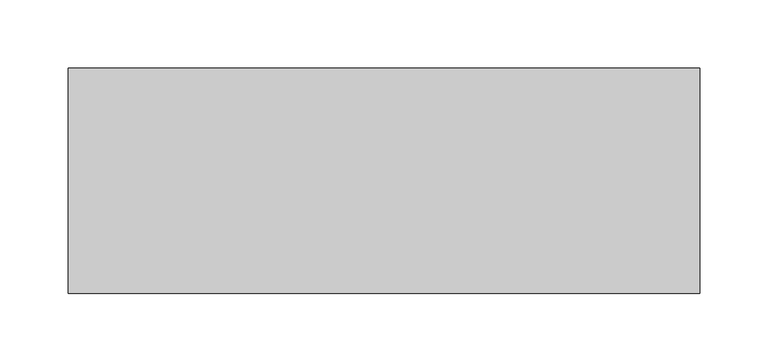
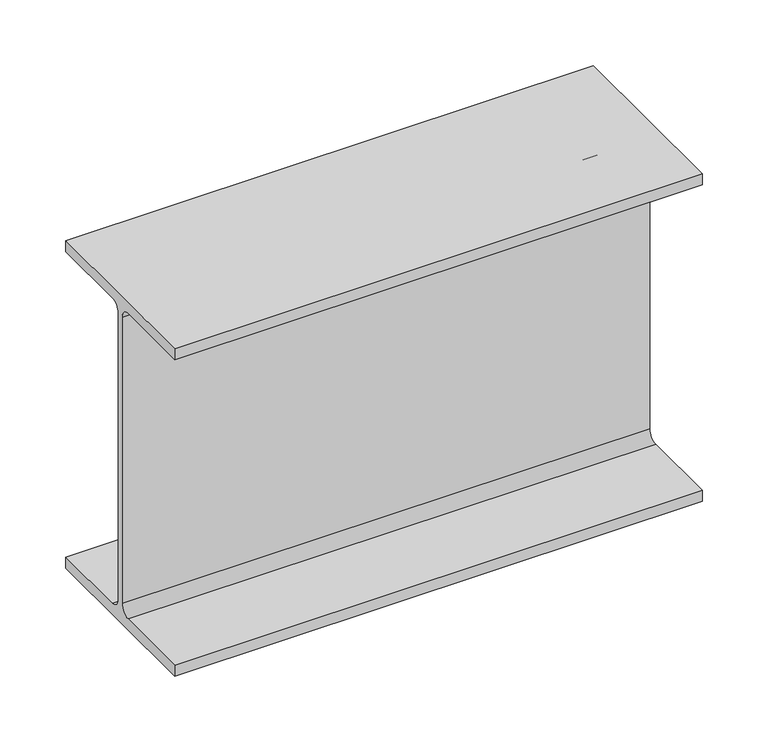
"""IFC4 building model written with IfcOpenShell, lengths in millimetres: beam geometry, Old_Steel Beam_H-KSD3502 : H_SB_ASB_H-300×150x6.5x9."""

import ifcopenshell
import ifcopenshell.guid

model = None  # the IFC model being written
_history = None  # IfcOwnerHistory: only IFC2X3 demands one
_inside = {}  # id of a spatial element -> (the spatial element, [elements in it])
_under = {}  # id of a project, library or spatial element -> (it, [spatial elements below it])
_declared = {}  # id of a project -> (the project, [libraries it declares])
_typed = {}  # id of a type object -> (the type object, [elements of that type])
_made_of = {}  # id of a material, layer set ... -> (it, [elements and type objects made of it])


def new_model(schema):
    """Start an empty IFC model of exactly this schema.

    Asked for "IFC4X3", IfcOpenShell would pick the latest addendum, in which some entities
    have other attributes; the version numbers below select the first issue.
    IFC2X3 requires an IfcOwnerHistory on every rooted entity: one is made here for all.
    """
    global model, _history
    if schema == "IFC4X3":
        model = ifcopenshell.file(schema_version=(4, 3, 0, 0))
    else:
        model = ifcopenshell.file(schema=schema)
    _inside.clear()
    _under.clear()
    _declared.clear()
    _typed.clear()
    _made_of.clear()
    _history = None
    if model.schema == "IFC2X3":
        org = make("IfcOrganization", Name="unknown")
        user = make(
            "IfcPersonAndOrganization",
            ThePerson=make("IfcPerson", FamilyName="unknown"),
            TheOrganization=org,
        )
        app = make(
            "IfcApplication",
            ApplicationDeveloper=org,
            Version="unknown",
            ApplicationFullName="unknown",
            ApplicationIdentifier="unknown",
        )
        _history = make(
            "IfcOwnerHistory",
            OwningUser=user,
            OwningApplication=app,
            ChangeAction="ADDED",
            CreationDate=0,
        )
    return model


def make(cls, **values):
    """One entity of the class cls with the attributes given. An attribute that is None is left unset."""
    return model.create_entity(
        cls, **{name: value for name, value in values.items() if value is not None}
    )


def rooted(cls, **values):
    """An entity with a GlobalId (a new one), such as an element, a storey or a relation."""
    return make(cls, GlobalId=ifcopenshell.guid.new(), OwnerHistory=_history, **values)


def si_unit(unit_type, name, prefix=None):
    """IfcSIUnit, for example si_unit("LENGTHUNIT", "METRE", prefix="MILLI")."""
    return make("IfcSIUnit", UnitType=unit_type, Prefix=prefix, Name=name)


def assignment(units):
    """IfcUnitAssignment: the units of a project."""
    return None if units is None else make("IfcUnitAssignment", Units=units)


def point(xyz):
    """IfcCartesianPoint."""
    return None if xyz is None else make("IfcCartesianPoint", Coordinates=xyz)


def direction(xyz):
    """IfcDirection."""
    return None if xyz is None else make("IfcDirection", DirectionRatios=xyz)


def frame(location, z_axis=None, x_axis=None):
    """IfcAxis2Placement3D, a coordinate frame: its origin and axes. An axis left out is left unset."""
    return make(
        "IfcAxis2Placement3D",
        Location=point(location),
        Axis=direction(z_axis),
        RefDirection=direction(x_axis),
    )


def frame_2d(location, x_axis=None):
    """IfcAxis2Placement2D, a coordinate frame in the plane: its origin and x axis."""
    return make(
        "IfcAxis2Placement2D", Location=point(location), RefDirection=direction(x_axis)
    )


def origin():
    """The frame at (0, 0, 0) with its axes left unset."""
    return frame((0.0, 0.0, 0.0))


def place(relative_to, where):
    """IfcLocalPlacement: puts the frame where relative to a parent placement (None: the world)."""
    return make(
        "IfcLocalPlacement", PlacementRelTo=relative_to, RelativePlacement=where
    )


def context(
    kind, dimensions, precision=None, world=None, true_north=None, identifier=None
):
    """IfcGeometricRepresentationContext, for example the 3D "Model" context."""
    return make(
        "IfcGeometricRepresentationContext",
        ContextIdentifier=identifier,
        ContextType=kind,
        CoordinateSpaceDimension=dimensions,
        Precision=precision,
        WorldCoordinateSystem=world,
        TrueNorth=true_north,
    )


def project(units=None, contexts=None):
    """IfcProject with its units and contexts."""
    return rooted(
        "IfcProject",
        Name="project",
        RepresentationContexts=contexts,
        UnitsInContext=assignment(units),
    )


def spatial(cls, under=None, at=None, **own):
    """A site, building, storey or space (cls), placed at a placement, below another one or the project."""
    s = rooted(cls, ObjectPlacement=at, **own)
    if under is not None:
        _under.setdefault(under.id(), (under, []))[1].append(s)
    return s


def polyline(points):
    """IfcPolyline through the points."""
    return make("IfcPolyline", Points=[point(p) for p in points])


def circle_curve(where, radius):
    """IfcCircle in the frame where."""
    return make("IfcCircle", Position=where, Radius=radius)


def trimmed(basis, trim1, trim2, sense, master):
    """IfcTrimmedCurve: the piece of a basis curve between two trims."""
    return make(
        "IfcTrimmedCurve",
        BasisCurve=basis,
        Trim1=trim1,
        Trim2=trim2,
        SenseAgreement=sense,
        MasterRepresentation=master,
    )


def segment(curve, same_sense, transition):
    """IfcCompositeCurveSegment."""
    return make(
        "IfcCompositeCurveSegment",
        Transition=transition,
        SameSense=same_sense,
        ParentCurve=curve,
    )


def composite_curve(segments, self_intersect=None):
    """IfcCompositeCurve: segments joined end to end."""
    return make("IfcCompositeCurve", Segments=segments, SelfIntersect=self_intersect)


def outline(outer, holes=None, kind="AREA"):
    """IfcArbitraryClosedProfileDef: a profile drawn as a closed curve; with holes, ...WithVoids."""
    if holes is None:
        return make("IfcArbitraryClosedProfileDef", ProfileType=kind, OuterCurve=outer)
    return make(
        "IfcArbitraryProfileDefWithVoids",
        ProfileType=kind,
        OuterCurve=outer,
        InnerCurves=holes,
    )


def extrude(swept, where, along, depth):
    """IfcExtrudedAreaSolid: the profile swept, set in the frame where, extruded along a direction by depth."""
    return make(
        "IfcExtrudedAreaSolid",
        SweptArea=swept,
        Position=where,
        ExtrudedDirection=direction(along),
        Depth=depth,
    )


def shape(context_of_items, identifier, shape_type, items):
    """IfcShapeRepresentation: the items that make up one representation, for example the "Body"."""
    return make(
        "IfcShapeRepresentation",
        ContextOfItems=context_of_items,
        RepresentationIdentifier=identifier,
        RepresentationType=shape_type,
        Items=items,
    )


def source(mapping_origin, context_of_items, identifier, shape_type, items):
    """IfcRepresentationMap: a shape defined once, which mapped items show again and again."""
    return make(
        "IfcRepresentationMap",
        MappingOrigin=mapping_origin,
        MappedRepresentation=shape(context_of_items, identifier, shape_type, items),
    )


def transform(
    local_origin,
    x_axis=None,
    y_axis=None,
    z_axis=None,
    scale=None,
    scale2=None,
    scale3=None,
    uniform=True,
):
    """IfcCartesianTransformationOperator3D, or its non-uniform kind. x_axis, y_axis, z_axis: its Axis1, 2, 3."""
    if uniform:
        return make(
            "IfcCartesianTransformationOperator3D",
            Axis1=direction(x_axis),
            Axis2=direction(y_axis),
            LocalOrigin=point(local_origin),
            Scale=scale,
            Axis3=direction(z_axis),
        )
    return make(
        "IfcCartesianTransformationOperator3DnonUniform",
        Axis1=direction(x_axis),
        Axis2=direction(y_axis),
        LocalOrigin=point(local_origin),
        Scale=scale,
        Axis3=direction(z_axis),
        Scale2=scale2,
        Scale3=scale3,
    )


def mapped(mapping_source, mapping_target):
    """IfcMappedItem: shows the shape of a source again, moved by a transform."""
    return make(
        "IfcMappedItem", MappingSource=mapping_source, MappingTarget=mapping_target
    )


def made_of(thing, what):
    """Note that an element or type object is made of a material, layer set ...; save() writes the relation."""
    if what is not None:
        _made_of.setdefault(what.id(), (what, []))[1].append(thing)
    return thing


def element(
    cls,
    number,
    at=None,
    inside=None,
    cuts=None,
    type_object=None,
    material=None,
    context=None,
    identifier="Body",
    shape_type=None,
    held_by="IfcProductDefinitionShape",
    body=None,
    shapes=None,
    **own,
):
    """One element of the class cls, such as IfcWall. Its Tag is "e" and its number.

    at: its placement. inside: the storey or other place that contains it. cuts: it is an
    opening in that element (IfcRelVoidsElement). A single representation is given by context,
    identifier, shape_type and body (its items); several are given by shapes. held_by: the class
    of the entity that holds the representations. save() writes the other relations.
    """
    e = rooted(cls, Tag="e%d" % number, ObjectPlacement=at, **own)
    if body is not None:
        shapes = [shape(context, identifier, shape_type, body)]
    if shapes is not None:
        e.Representation = make(held_by, Representations=shapes)
    if inside is not None:
        _inside.setdefault(inside.id(), (inside, []))[1].append(e)
    if cuts is not None:
        rooted(
            "IfcRelVoidsElement", RelatingBuildingElement=cuts, RelatedOpeningElement=e
        )
    if type_object is not None:
        _typed.setdefault(type_object.id(), (type_object, []))[1].append(e)
    return made_of(e, material)


def aggregate(whole, parts):
    """IfcRelAggregates: a whole, such as a stair, and the parts it consists of."""
    return rooted("IfcRelAggregates", RelatingObject=whole, RelatedObjects=parts)


def save(model, path):
    """Write the relations noted so far, then the file.

    IfcRelAggregates (storeys below a building ...), IfcRelContainedInSpatialStructure (elements
    in a storey), IfcRelDefinesByType, IfcRelAssociatesMaterial and IfcRelDeclares: one each for
    every whole, place, type object, material and project.
    """
    for whole, parts in _under.values():
        aggregate(whole, parts)
    for where, things in _inside.values():
        rooted(
            "IfcRelContainedInSpatialStructure",
            RelatedElements=things,
            RelatingStructure=where,
        )
    for kind, things in _typed.values():
        rooted("IfcRelDefinesByType", RelatedObjects=things, RelatingType=kind)
    for what, things in _made_of.values():
        rooted("IfcRelAssociatesMaterial", RelatedObjects=things, RelatingMaterial=what)
    for by, libraries in _declared.values():
        rooted("IfcRelDeclares", RelatingContext=by, RelatedDefinitions=libraries)
    model.write(path)


def beam_c8f6394c(model_context):
    return source(origin(), model_context, "Body", "SweptSolid", [
        extrude(outline(composite_curve([segment(polyline([(82.5, -141.5), (82.5, -151.7), (-82.5, -151.7), (-82.5, -141.5), (-11.9, -141.5)]), True, "CONTINUOUS"), segment(trimmed(circle_curve(frame_2d((-11.9, -132.6)), 8.9), [point((-11.9, -141.5))], [point((-3.0, -132.6))], True, "CARTESIAN"), True, "CONTINUOUS"), segment(polyline([(-3.0, -132.6), (-3.0, 132.6)]), True, "CONTINUOUS"), segment(trimmed(circle_curve(frame_2d((-11.9, 132.6)), 8.9), [point((-3.0, 132.6))], [point((-11.9, 141.5))], True, "CARTESIAN"), True, "CONTINUOUS"), segment(polyline([(-11.9, 141.5), (-82.5, 141.5), (-82.5, 151.7), (82.5, 151.7), (82.5, 141.5), (11.9, 141.5)]), True, "CONTINUOUS"), segment(trimmed(circle_curve(frame_2d((11.9, 132.6)), 8.9), [point((11.9, 141.5))], [point((3.0, 132.6))], True, "CARTESIAN"), True, "CONTINUOUS"), segment(polyline([(3.0, 132.6), (3.0, -132.6)]), True, "CONTINUOUS"), segment(trimmed(circle_curve(frame_2d((11.9, -132.6)), 8.9), [point((3.0, -132.6))], [point((11.9, -141.5))], True, "CARTESIAN"), True, "CONTINUOUS"), segment(polyline([(11.9, -141.5), (82.5, -141.5)]), True, "CONTINUOUS")], self_intersect=False)), frame((-300.0, 0.0, 0.0), z_axis=(1.0, 0.0, 0.0), x_axis=(0.0, 1.0, 0.0)), (0.0, 0.0, 1.0), 462.3),
    ])


if __name__ == "__main__":
    model = new_model("IFC4")
    model_context = context("Model", 3, world=origin())
    ifc_project = project(units=[si_unit("LENGTHUNIT", "METRE", prefix="MILLI")], contexts=[model_context])
    site = spatial("IfcSite", under=ifc_project)
    building = spatial("IfcBuilding", under=site)
    placement = place(None, origin())
    beam_shape = beam_c8f6394c(model_context)
    element("IfcBeam", 1, ObjectType="Old_Steel Beam_H-KSD3502 : H_SB_ASB_H-300×150x6.5x9", at=placement, inside=building, context=model_context, shape_type="MappedRepresentation", body=[
        mapped(beam_shape, transform((0.0, 0.0, 0.0), x_axis=(1.0, 0.0, 0.0), y_axis=(0.0, 1.0, 0.0), z_axis=(0.0, 0.0, 1.0))),
    ])
    save(model, "model.ifc")

# Revit data of these elements
# Type "Old_Steel Beam_H-KSD3502 : H_SB_ASB_H-300×150x6.5x9"
#   Width = 15.0 cm
#   Web Thickness = 0.65 cm
#   Web Fillet = 1.3 cm
#   Warping Constant = 107174.0 cm⁶
#   Torsional Moment of Inertia = 9.9539 cm⁴
#   Torsional Modulus = 1.0 cm³
#   Section Area = 46.78 cm²
#   Plastic Modulus weak axis = 105.0 cm³
#   Plastic Modulus strong axis = 542.0 cm³
#   Perimeter = 1.17 m²/m
#   Nominal Weight = 36.70 kgf/m
#   Moment of Inertia weak axis = 508.00 cm⁴
#   Moment of Inertia strong axis = 7210.00 cm⁴
#   Height = 30.0 cm
#   Flange Thickness = 0.9 cm
#   Elastic Modulus weak axis = 67.7 cm³
#   Elastic Modulus strong axis = 481.0 cm³
#   Centroid Vertical = 15.0 cm
#   Centroid Horizontal = 7.5 cm
#   Length [instance default] = 1.5240 m
#   Structural Material [instance default] = Steel, 45-345
#   Assembly Code = ""
# Element 1 (IfcBeam, "Old_Steel Beam_H-KSD3502 : H_SB_ASB_H-300×150x6.5x9")
#   Structural Material = none
# Materials
#   "Steel, 45-345": class "Metal", colour RGB 189 187 185, transparency 0, Description = "Steel 345 MPa", Cost = 0
